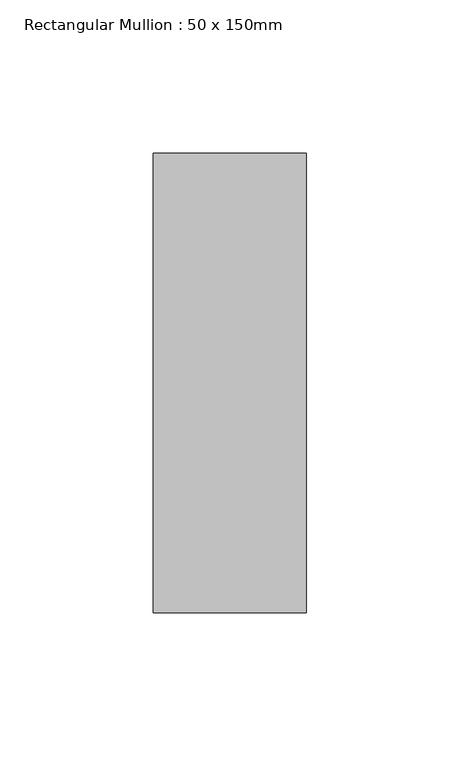
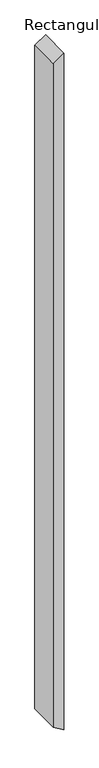
"""IFC4 building model written with IfcOpenShell, lengths in millimetres: member geometry, Rectangular Mullion : 50 x 150mm."""

from ifc_helpers import new_model, si_unit, frame, origin, place, context, project, spatial, polyline, outline, extrude, source, transform, mapped, element, save


def rectangular_mullion_50_x_150mm_82bd072a(model_context):
    return source(origin(), model_context, "Body", "SweptSolid", [
        extrude(outline(polyline([(0.0, 0.0), (-34.9055374, -50.0), (-3342.3079561, -50.0), (-3371.6090252, 0.0), (0.0, 0.0)])), frame((0.0, -75.0, 0.0), z_axis=(0.0, 1.0, 0.0), x_axis=(0.0, 0.0, 1.0)), (0.0, 0.0, 1.0), 150.0),
    ])


if __name__ == "__main__":
    model = new_model("IFC4")
    model_context = context("Model", 3, world=origin())
    ifc_project = project(units=[si_unit("LENGTHUNIT", "METRE", prefix="MILLI")], contexts=[model_context])
    site = spatial("IfcSite", under=ifc_project)
    building = spatial("IfcBuilding", under=site)
    placement = place(None, origin())
    rectangular_mullion_50_x_150mm_shape = rectangular_mullion_50_x_150mm_82bd072a(model_context)
    element("IfcMember", 1, ObjectType="Rectangular Mullion : 50 x 150mm", at=placement, inside=building, context=model_context, shape_type="MappedRepresentation", body=[
        mapped(rectangular_mullion_50_x_150mm_shape, transform((0.0, 0.0, 0.0), x_axis=(1.0, 0.0, 0.0), y_axis=(0.0, 1.0, 0.0), z_axis=(0.0, 0.0, 1.0))),
    ])
    save(model, "model.ifc")

# Revit data of these elements
# Type "Rectangular Mullion : 50 x 150mm"
#   built-in parameter 1007304 = 0.492126 (stored number, unit not read)
#   built-in parameter 1007301 = 0.082021 (stored number, unit not read)
#   built-in parameter 1007300 = 0.082021 (stored number, unit not read)
# Element 1 (IfcMember, "Rectangular Mullion : 50 x 150mm")
#   Materials on its faces: "Metal - Aluminium"
# Materials
#   "Metal - Aluminium": class "Metal", colour RGB 247 247 247, transparency 0
